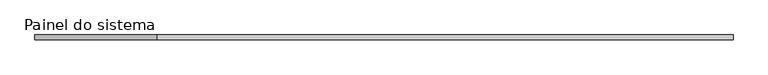
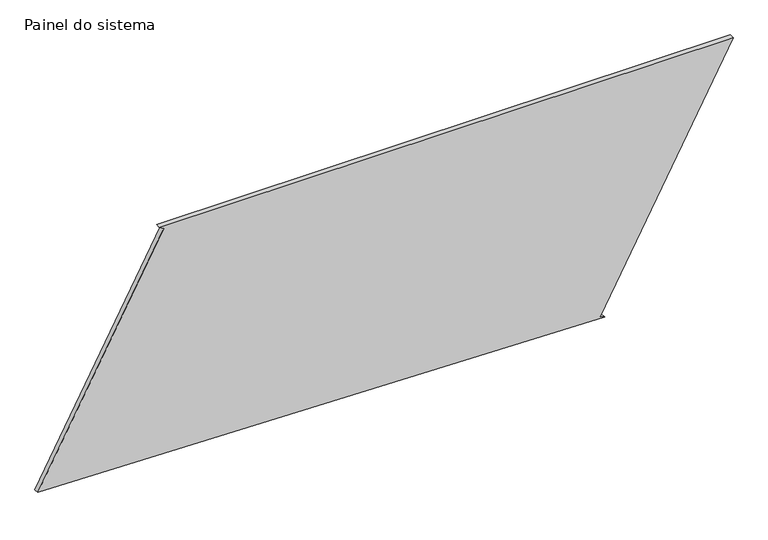
"""IFC4 building model written with IfcOpenShell, lengths in millimetres: plate geometry, Painel do sistema : Envidraçado."""

from ifc_helpers import new_model, si_unit, frame, origin, place, context, project, spatial, polyline, outline, extrude, source, transform, mapped, element, save


def painel_do_sistema_89a5c3f4(model_context):
    return source(origin(), model_context, "Body", "SweptSolid", [
        extrude(outline(polyline([(0.0, 1103.733258), (11.7958757, 1081.6910867), (1262.5400637, 1751.0272739), (1262.5400637, -1138.4667994), (1250.744188, -1116.4246281), (64.9042677, -1751.0272739), (0.0, 1103.733258)])), frame((0.0, 24.5, 0.0), z_axis=(0.0, 1.0, 0.0), x_axis=(0.0, 0.0, 1.0)), (0.0, 0.0, 1.0), 25.0),
    ])


if __name__ == "__main__":
    model = new_model("IFC4")
    model_context = context("Model", 3, world=origin())
    ifc_project = project(units=[si_unit("LENGTHUNIT", "METRE", prefix="MILLI")], contexts=[model_context])
    site = spatial("IfcSite", under=ifc_project)
    building = spatial("IfcBuilding", under=site)
    placement = place(None, origin())
    painel_do_sistema_shape = painel_do_sistema_89a5c3f4(model_context)
    element("IfcPlate", 1, ObjectType="Painel do sistema : Envidraçado", at=placement, inside=building, context=model_context, shape_type="MappedRepresentation", body=[
        mapped(painel_do_sistema_shape, transform((0.0, 0.0, 0.0), x_axis=(1.0, 0.0, 0.0), y_axis=(0.0, 1.0, 0.0), z_axis=(0.0, 0.0, 1.0))),
    ])
    save(model, "model.ifc")

# Revit data of these elements
# Type "Painel do sistema : Envidraçado"
#   Construction Type Id = "GSP4R"
#   Analytic Construction = "Vidraça única Pilkington 1/8 pol"
#   Visual Light Transmittance = 0.9
#   Solar Heat Gain Coefficient = 0.86
#   Heat Transfer Coefficient (U) = 6.7069 W/(m²·K)
# Element 1 (IfcPlate, "Painel do sistema : Envidraçado")
#   Materials on its faces: "Vidro"
# Materials
#   "Vidro": class "Vidro", colour RGB 0 128 192, transparency 0.9, Description = "Vidro de sílica", Cost = 0
